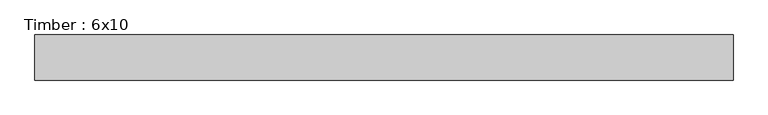
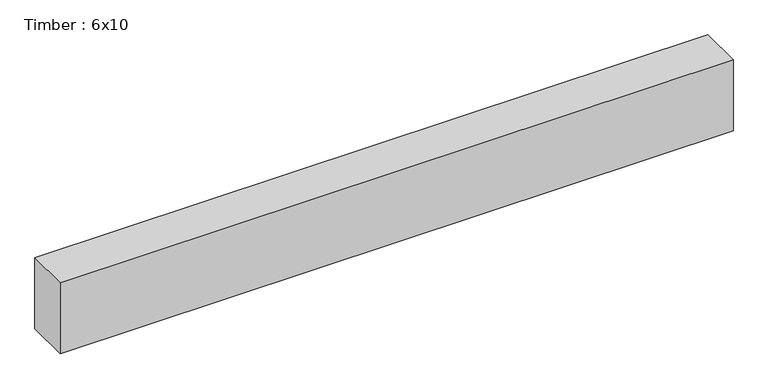
"""IFC4 building model written with IfcOpenShell, lengths in millimetres: beam geometry, Timber : 6x10."""

from ifc_helpers import new_model, si_unit, frame, origin, place, context, project, spatial, polyline, outline, extrude, source, transform, mapped, element, save


def timber_6x10_702de74f(model_context):
    return source(origin(), model_context, "Body", "SweptSolid", [
        extrude(outline(polyline([(1096.3279, 69.85), (1096.3279, -69.85), (-1065.1814977, -69.85), (-1065.1814977, 69.85), (1096.3279, 69.85)])), frame((0.0, 0.0, -120.65), z_axis=(0.0, 0.0, 1.0), x_axis=(1.0, 0.0, 0.0)), (0.0, 0.0, 1.0), 241.3),
    ])


if __name__ == "__main__":
    model = new_model("IFC4")
    model_context = context("Model", 3, world=origin())
    ifc_project = project(units=[si_unit("LENGTHUNIT", "METRE", prefix="MILLI")], contexts=[model_context])
    site = spatial("IfcSite", under=ifc_project)
    building = spatial("IfcBuilding", under=site)
    placement = place(None, origin())
    timber_6x10_shape = timber_6x10_702de74f(model_context)
    element("IfcBeam", 1, ObjectType="Timber : 6x10", at=placement, inside=building, context=model_context, shape_type="MappedRepresentation", body=[
        mapped(timber_6x10_shape, transform((0.0, 0.0, 0.0), x_axis=(1.0, 0.0, 0.0), y_axis=(0.0, 1.0, 0.0), z_axis=(0.0, 0.0, 1.0))),
    ])
    save(model, "model.ifc")

# Revit data of these elements
# Type "Timber : 6x10"
#   Assembly Code = "B10"
#   A = 0.362847 SF
#   Length [instance default] = 5' - 0"
#   b = 0' - 5 1/2"
#   d = 0' - 9 1/2"
#   Structural Material [instance default] = Softwood, Lumber
# Element 1 (IfcBeam, "Timber : 6x10")
#   Materials on its faces: "Softwood, Lumber"
# Materials
#   "Softwood, Lumber": class "Wood", colour RGB 144 113 62, transparency 0, Description = "Pinus Echinata", Cost = 0
